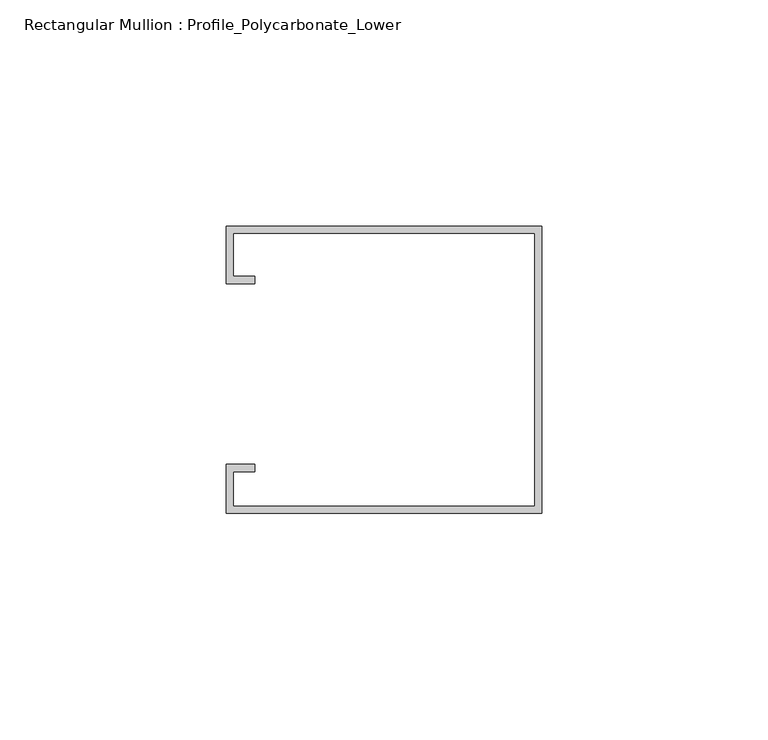
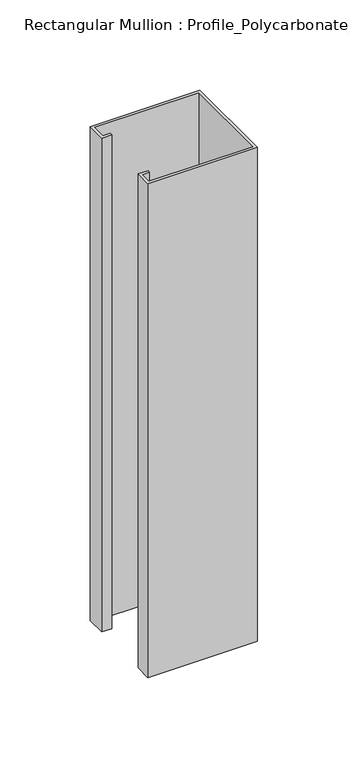
"""IFC4 building model written with IfcOpenShell, lengths in millimetres: member geometry, Rectangular Mullion : Profile_Polycarbonate_Lower."""

from ifc_helpers import new_model, si_unit, frame, origin, place, context, project, spatial, polyline, outline, extrude, source, transform, mapped, element, save


def rectangular_mullion_profile_polycarbonate_lower_45da0f66(model_context):
    return source(origin(), model_context, "Body", "SweptSolid", [
        extrude(outline(polyline([(0.0, 32.7), (0.0, -30.8), (-69.85, -30.8), (-69.85, -20.0), (-63.5, -20.0), (-63.5, -21.5875), (-68.2625, -21.5875), (-68.2625, -29.2125), (-1.5875, -29.2125), (-1.5875, 31.1125), (-68.2625, 31.1125), (-68.2625, 21.5875), (-63.5, 21.5875), (-63.5, 20.0), (-69.85, 20.0), (-69.85, 32.7), (0.0, 32.7)])), frame((0.0, 0.0, -333.375), z_axis=(0.0, 0.0, 1.0), x_axis=(1.0, 0.0, 0.0)), (0.0, 0.0, 1.0), 333.375),
    ])


if __name__ == "__main__":
    model = new_model("IFC4")
    model_context = context("Model", 3, world=origin())
    ifc_project = project(units=[si_unit("LENGTHUNIT", "METRE", prefix="MILLI")], contexts=[model_context])
    site = spatial("IfcSite", under=ifc_project)
    building = spatial("IfcBuilding", under=site)
    placement = place(None, origin())
    rectangular_mullion_profile_polycarbonate_lower_shape = rectangular_mullion_profile_polycarbonate_lower_45da0f66(model_context)
    element("IfcMember", 1, ObjectType="Rectangular Mullion : Profile_Polycarbonate_Lower", at=placement, inside=building, context=model_context, shape_type="MappedRepresentation", body=[
        mapped(rectangular_mullion_profile_polycarbonate_lower_shape, transform((0.0, 0.0, 0.0), x_axis=(1.0, 0.0, 0.0), y_axis=(0.0, 1.0, 0.0), z_axis=(0.0, 0.0, 1.0))),
    ])
    save(model, "model.ifc")

# Revit data of these elements
# Type "Rectangular Mullion : Profile_Polycarbonate_Lower"
#   built-in parameter 1007322 = 0.208333 (stored number, unit not read)
#   built-in parameter 1007321 = 0 (stored number, unit not read)
#   built-in parameter 1007320 = 0.00520833 (stored number, unit not read)
# Element 1 (IfcMember, "Rectangular Mullion : Profile_Polycarbonate_Lower")
#   Materials on its faces: "GALVANIZED UNISTRUT P5500, 1 5/8\" X 2 7/16\" OR ALUM. CHANNEL"
# Materials
#   "GALVANIZED UNISTRUT P5500, 1 5/8\" X 2 7/16\" OR ALUM. CHANNEL": class "Metal", colour RGB 244 244 244, transparency 0, Description = "Aluminum 6061", Cost = 0
